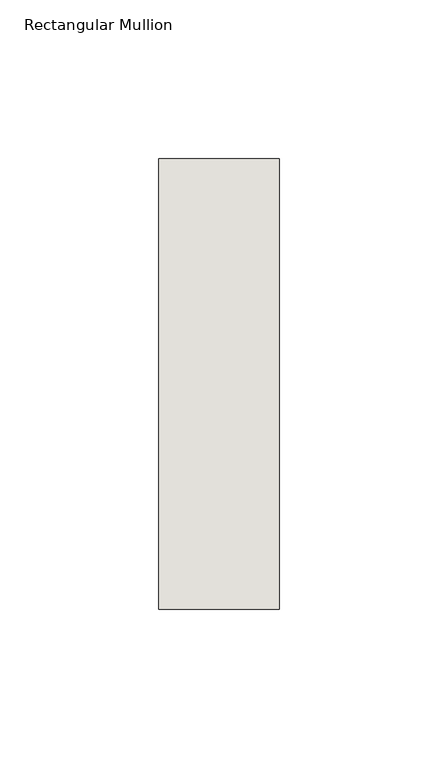
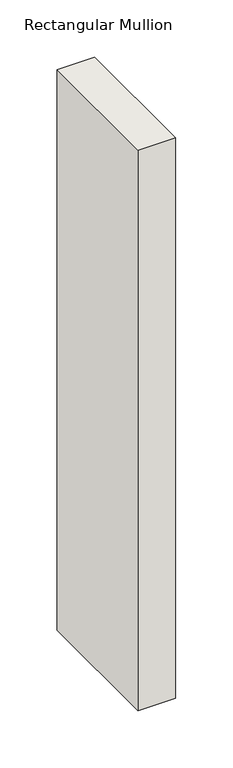
"""IFC4 building model written with IfcOpenShell, lengths in millimetres: wall geometry, Rectangular Mullion : NLRS_21_CWM_hsb-regel 38x142_gen_rsf."""

from ifc_helpers import new_model, si_unit, frame, origin, place, context, project, spatial, polyline, outline, extrude, source, transform, mapped, element, save


def rectangular_mullion_45531403(model_context):
    return source(origin(), model_context, "Body", "SweptSolid", [
        extrude(outline(polyline([(19.0, -71.0), (-19.0, -71.0), (-19.0, 71.0), (19.0, 71.0), (19.0, -71.0)])), frame((0.0, 0.0, -599.0), z_axis=(0.0, 0.0, 1.0), x_axis=(1.0, 0.0, 0.0)), (0.0, 0.0, 1.0), 599.0),
    ])


if __name__ == "__main__":
    model = new_model("IFC4")
    model_context = context("Model", 3, world=origin())
    ifc_project = project(units=[si_unit("LENGTHUNIT", "METRE", prefix="MILLI")], contexts=[model_context])
    site = spatial("IfcSite", under=ifc_project)
    building = spatial("IfcBuilding", under=site)
    placement = place(None, origin())
    rectangular_mullion_shape = rectangular_mullion_45531403(model_context)
    element("IfcWall", 1, ObjectType="Rectangular Mullion : NLRS_21_CWM_hsb-regel 38x142_gen_rsf", at=placement, inside=building, context=model_context, shape_type="MappedRepresentation", body=[
        mapped(rectangular_mullion_shape, transform((0.0, 0.0, 0.0), x_axis=(1.0, 0.0, 0.0), y_axis=(0.0, 1.0, 0.0), z_axis=(0.0, 0.0, 1.0))),
    ])
    save(model, "model.ifc")

# Revit data of these elements
# Type "Rectangular Mullion : NLRS_21_CWM_hsb-regel 38x142_gen_rsf"
#   Type IfcGUID = "07M7mRoiH1CR8m_RSKIwpF"
#   Assembly Code = "21.10"
#   IfcExportAs = "IfcWall"
#   built-in parameter 1007322 = 0.465879 (stored number, unit not read)
#   built-in parameter 1007321 = 0.062336 (stored number, unit not read)
#   built-in parameter 1007320 = 0.062336 (stored number, unit not read)
# Element 1 (IfcWall, "Rectangular Mullion : NLRS_21_CWM_hsb-regel 38x142_gen_rsf")
#   Materials on its faces: "NLRS_i2_hout naaldhout vuren_gen_rsf"
# Materials
#   "NLRS_i2_hout naaldhout vuren_gen_rsf": class "I - Hout", colour RGB 234 199 147, transparency 0, Keynote = "i2", Manufacturer = "Revit Standards Foundation", URL = "www.revitstandards.org", Description = "hout vuren", Cost = 0
